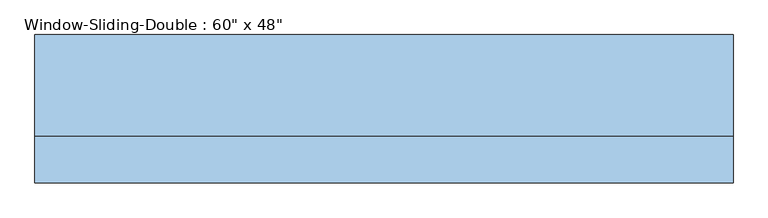
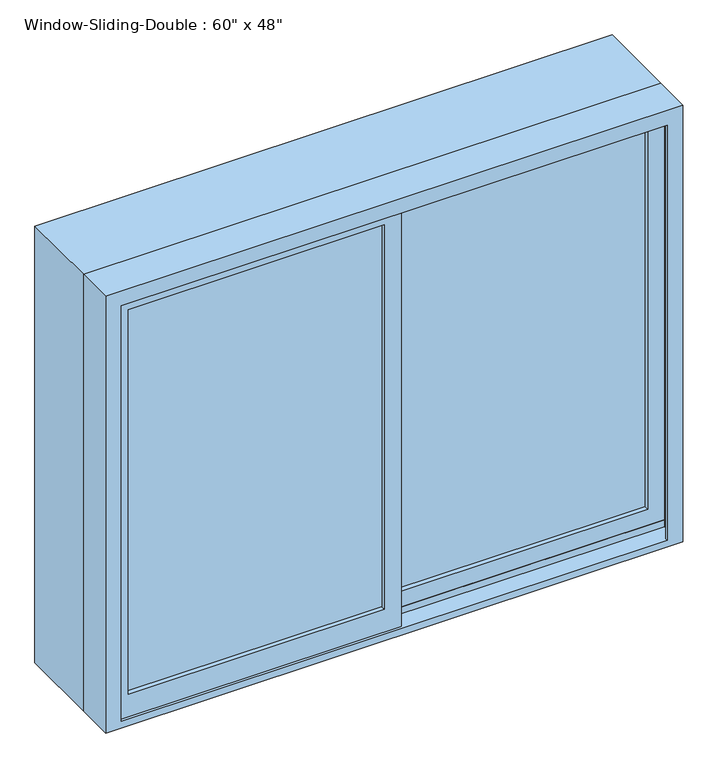
"""IFC4 building model written with IfcOpenShell, lengths in millimetres: window geometry."""

from ifc_helpers import new_model, si_unit, frame, origin, place, context, project, spatial, polyline, outline, extrude, faceted_brep, source, transform, mapped, element, save


def window_6e1e4071(model_context):
    return source(origin(), model_context, "Body", "SolidModel", [
        faceted_brep([(-762.0, -66.04, 914.4), (762.0, -66.04, 914.4), (762.0, -167.64, 914.4), (-762.0, -167.64, 914.4), (-721.0778905, -167.64, 2092.6778905), (-721.0778905, -167.64, 933.45), (-721.0778905, -161.29, 933.45), (-721.0778905, -161.29, 2092.6778905), (-742.95, -161.29, 933.45), (-742.95, -161.29, 2114.55), (742.95, -161.29, 2114.55), (742.95, -161.29, 933.45), (721.0778905, -161.29, 933.45), (721.0778905, -161.29, 2092.6778905), (-742.95, -116.84, 933.45), (-742.95, -116.84, 952.5), (-742.95, -72.39, 952.5), (-742.95, -72.39, 933.45), (-742.95, -66.04, 933.45), (-742.95, -66.04, 2114.55), (-762.0, -66.04, 2133.6), (762.0, -66.04, 2133.6), (742.95, -66.04, 2114.55), (742.95, -66.04, 933.45), (-762.0, -167.64, 2133.6), (762.0, -167.64, 2133.6), (721.0778905, -167.64, 2092.6778905), (721.0778905, -167.64, 933.45), (742.95, -72.39, 933.45), (742.95, -72.39, 952.5), (742.95, -116.84, 952.5), (742.95, -116.84, 933.45)], [[[0, 1, 2, 3]], [[4, 5, 6, 7]], [[7, 6, 8, 9, 10, 11, 12, 13]], [[9, 8, 14, 15, 16, 17, 18, 19]], [[0, 20, 21, 1], [22, 19, 18, 23]], [[24, 20, 0, 3]], [[2, 25, 24, 3], [4, 26, 27, 5]], [[7, 13, 26, 4]], [[9, 19, 22, 10]], [[20, 24, 25, 21]], [[13, 12, 27, 26]], [[22, 23, 28, 29, 30, 31, 11, 10]], [[21, 25, 2, 1]], [[27, 12, 11, 31, 14, 8, 6, 5]], [[31, 30, 15, 14]], [[30, 29, 16, 15]], [[29, 28, 17, 16]], [[18, 17, 28, 23]]]),
        extrude(outline(polyline([(2133.6, 762.0), (2133.6, -762.0), (914.4, -762.0), (914.4, 762.0), (2133.6, 762.0)]), holes=[polyline([(2114.55, -742.95), (2114.55, 742.95), (933.45, 742.95), (933.45, -742.95), (2114.55, -742.95)])]), frame((0.0, -66.04, 0.0), z_axis=(0.0, 1.0, 0.0), x_axis=(0.0, 0.0, 1.0)), (0.0, 0.0, 1.0), 222.25),
        extrude(outline(polyline([(698.5, -104.14), (22.225, -104.14), (22.225, -97.79), (698.5, -97.79), (698.5, -104.14)])), frame((0.0, 0.0, 996.95), z_axis=(0.0, 0.0, 1.0), x_axis=(1.0, 0.0, 0.0)), (0.0, 0.0, 1.0), 1073.15),
        extrude(outline(polyline([(698.5, -91.44), (22.225, -91.44), (22.225, -85.09), (698.5, -85.09), (698.5, -91.44)])), frame((0.0, 0.0, 996.95), z_axis=(0.0, 0.0, 1.0), x_axis=(1.0, 0.0, 0.0)), (0.0, 0.0, 1.0), 1073.15),
        extrude(outline(polyline([(-22.225, -148.59), (-698.5, -148.59), (-698.5, -142.24), (-22.225, -142.24), (-22.225, -148.59)])), frame((0.0, 0.0, 996.95), z_axis=(0.0, 0.0, 1.0), x_axis=(1.0, 0.0, 0.0)), (0.0, 0.0, 1.0), 1073.15),
        extrude(outline(polyline([(-22.225, -135.89), (-698.5, -135.89), (-698.5, -129.54), (-22.225, -129.54), (-22.225, -135.89)])), frame((0.0, 0.0, 996.95), z_axis=(0.0, 0.0, 1.0), x_axis=(1.0, 0.0, 0.0)), (0.0, 0.0, 1.0), 1073.15),
        extrude(outline(polyline([(933.45, 22.225), (2114.55, 22.225), (2114.55, -742.95), (933.45, -742.95), (933.45, 22.225)]), holes=[polyline([(2070.1, -698.5), (2070.1, -22.225), (996.95, -22.225), (996.95, -698.5), (2070.1, -698.5)])]), frame((0.0, -161.29, 0.0), z_axis=(0.0, 1.0, 0.0), x_axis=(0.0, 0.0, 1.0)), (0.0, 0.0, 1.0), 44.45),
        extrude(outline(polyline([(952.5, -22.225), (952.5, 742.95), (2114.55, 742.95), (2114.55, -22.225), (952.5, -22.225)]), holes=[polyline([(996.95, 698.5), (996.95, 22.225), (2070.1, 22.225), (2070.1, 698.5), (996.95, 698.5)])]), frame((0.0, -116.84, 0.0), z_axis=(0.0, 1.0, 0.0), x_axis=(0.0, 0.0, 1.0)), (0.0, 0.0, 1.0), 44.45),
    ])


if __name__ == "__main__":
    model = new_model("IFC4")
    model_context = context("Model", 3, world=origin())
    ifc_project = project(units=[si_unit("LENGTHUNIT", "METRE", prefix="MILLI")], contexts=[model_context])
    site = spatial("IfcSite", under=ifc_project)
    building = spatial("IfcBuilding", under=site)
    placement = place(None, origin())
    window_shape = window_6e1e4071(model_context)
    element("IfcWindow", 1, ObjectType="Window-Sliding-Double : 60\" x 48\"", at=placement, inside=building, context=model_context, shape_type="MappedRepresentation", body=[
        mapped(window_shape, transform((0.0, 0.0, 0.0), x_axis=(1.0, 0.0, 0.0), y_axis=(0.0, 1.0, 0.0), z_axis=(0.0, 0.0, 1.0))),
    ])
    save(model, "model.ifc")

# Revit data of these elements
# Project information
#   Organization Name = "G3B Press"
#   Organization Description = "Paul F. Aubin Cosulting Services, Inc."
#   Building Name = "Revit Essentials for Architecture"
#   Author = "Paul F. Aubin"
#   Author Website = "https://www.paulaubin.com"
#   Copyright = "Copyright © 2020 Paul F Aubin, all rights reserved"
#   Project Issue Date = "8/1/2020"
#   Project Status = "Schematic Design"
#   Client Name = "Groups and Links"
#   Project Address = "Enter address here"
#   Project Name = "Understanding Groups"
#   Project Number = "2020.05A"
# Type "Window-Sliding-Double : 60\" x 48\""
#   Type Mark = "A"
#   Fire Rating = "0.5h"
#   Assembly Code = "B2020100"
#   Analytic Construction = "Double glazing - domestic"
#   Window Inset [instance default] = 0' - 0"
#   Wall Thickness [instance default] = 0' - 6"
#   Visual Light Transmittance = 0.81
#   Thermal Resistance (R) = 1.8146 (h·ft²·°F)/BTU
#   Solar Heat Gain Coefficient = 0.76
#   Muntin Width = 2' - 2 5/8"
#   Muntin Height = 3' - 6 1/4"
#   Interior Wall Closure [instance default] = 0' - 2 3/4"
#   Heat Transfer Coefficient (U) = 0.5511 BTU/(h·ft²·°F)
#   Frame Extension [instance default] = 0' - 0 1/4"
#   Exterior Wall Closure [instance default] = 0' - 1 1/4"
#   Rough Width = 5' - 0 1/2"
#   Rough Height = 4' - 0 1/2"
#   Height = 4' - 0"
#   Extension Jamb [instance default] = 0' - 2 3/4"
#   Default Sill Height = 3' - 0"
#   Width = 5' - 0"
#   Interior Trim Visibility [instance default] = yes
#   Indicator Visibility [instance default] = yes
#   Exterior Trim Visibility [instance default] = yes
#   Muntin Visibility = yes
#   Extension Jamb Visibility [instance default] = yes
#   Muntin Pattern = Muntin Pattern_2x2 : Muntin Pattern_2x2
#   Interior Trim Material = Cherry
#   Interior Trim = Trim-Window-Interior-Flat : Picture Frame
#   Interior Frame Material = Cherry
#   Glass Panel Material = Glass, Clear Glazing
#   Exterior Trim Material = PVC, Flexible
#   Exterior Trim = Trim-Window-Exterior-Flat : with Sill
#   Exterior Frame Material = PVC, Flexible
#   Wall Closure = (empty or 0)
# Element 1 (IfcWindow, "Window-Sliding-Double : 60\" x 48\"")
#   Wall Thickness = 1' - 0"
#   Extension Jamb = 0' - 8 3/4"
#   Materials on its faces: "Cherry", "Glass, Clear Glazing", "PVC, Flexible"
# Materials
#   "Cherry": class "Wood", colour RGB 157 77 38, transparency 0, Description = "Prunus Serotina", Cost = 0
#   "Glass, Clear Glazing": class "Glass", colour RGB 120 120 120, transparency 0, Description = "Clear glazing", Cost = 0
#   "PVC, Flexible": class "Plastic", colour RGB 178 178 178, transparency 0, Description = "Flexible polyvinyl chloride", Cost = 0
